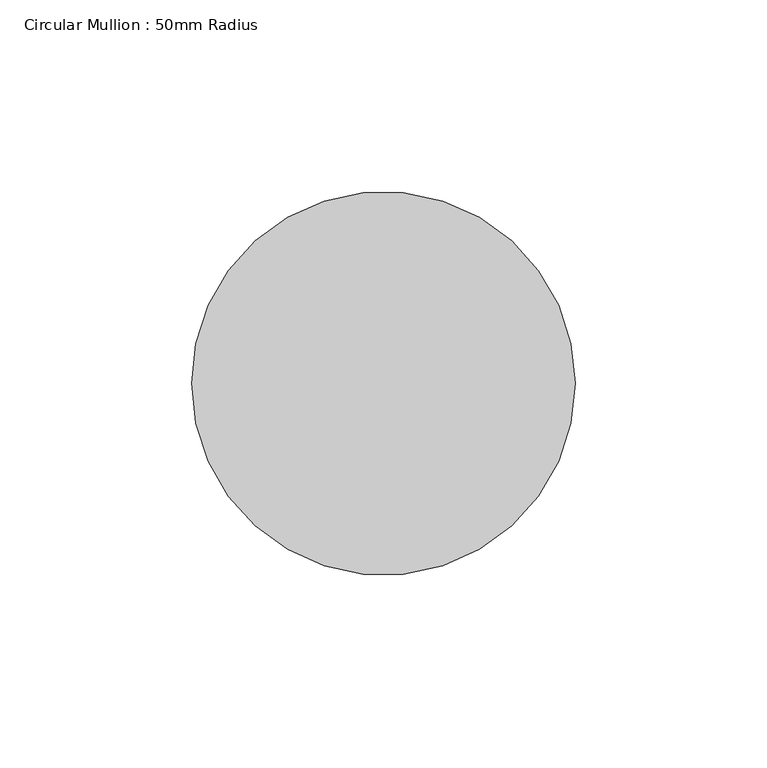
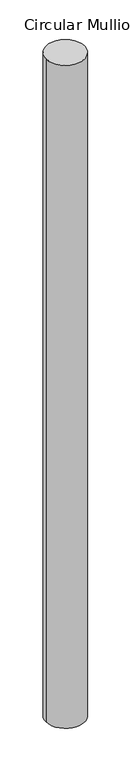
"""IFC4 building model written with IfcOpenShell, lengths in millimetres: member geometry, Circular Mullion : 50mm Radius."""

from ifc_helpers import new_model, si_unit, point, frame, origin, origin_2d, place, context, project, spatial, circle_curve, trimmed, segment, composite_curve, outline, extrude, source, transform, mapped, element, save


def circular_mullion_50mm_radius_254c7490(model_context):
    return source(origin(), model_context, "Body", "SweptSolid", [
        extrude(outline(composite_curve([segment(trimmed(circle_curve(origin_2d(), 50.0), [point((50.0, 0.0))], [point((-50.0, 0.0))], False, "CARTESIAN"), True, "CONTINUOUS"), segment(trimmed(circle_curve(origin_2d(), 50.0), [point((-50.0, 0.0))], [point((50.0, 0.0))], False, "CARTESIAN"), True, "CONTINUOUS")], self_intersect=False)), frame((0.0, 0.0, -1802.5662254), z_axis=(0.0, 0.0, 1.0), x_axis=(1.0, 0.0, 0.0)), (0.0, 0.0, 1.0), 1802.5662254),
    ])


if __name__ == "__main__":
    model = new_model("IFC4")
    model_context = context("Model", 3, world=origin())
    ifc_project = project(units=[si_unit("LENGTHUNIT", "METRE", prefix="MILLI")], contexts=[model_context])
    site = spatial("IfcSite", under=ifc_project)
    building = spatial("IfcBuilding", under=site)
    placement = place(None, origin())
    circular_mullion_50mm_radius_shape = circular_mullion_50mm_radius_254c7490(model_context)
    element("IfcMember", 1, ObjectType="Circular Mullion : 50mm Radius", at=placement, inside=building, context=model_context, shape_type="MappedRepresentation", body=[
        mapped(circular_mullion_50mm_radius_shape, transform((0.0, 0.0, 0.0), x_axis=(1.0, 0.0, 0.0), y_axis=(0.0, 1.0, 0.0), z_axis=(0.0, 0.0, 1.0))),
    ])
    save(model, "model.ifc")

# Revit data of these elements
# Type "Circular Mullion : 50mm Radius"
#   built-in parameter 1007350 = 0.164042 (stored number, unit not read)
# Element 1 (IfcMember, "Circular Mullion : 50mm Radius")
#   Materials on its faces: "Aluminium"
# Materials
#   "Aluminium": class "Metal", colour RGB 247 247 247, transparency 0, Description = "Aluminium 6061", Cost = 0
